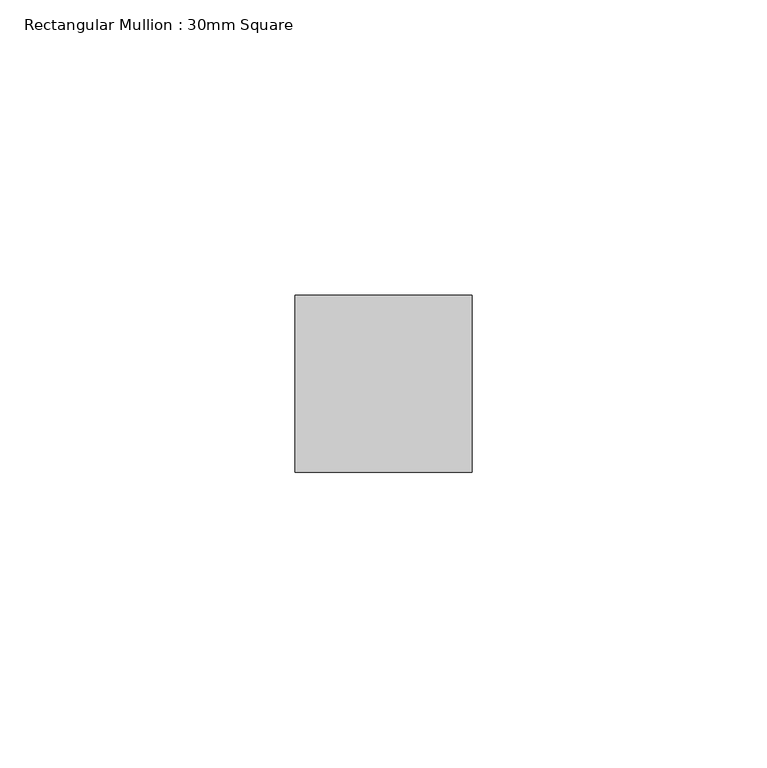
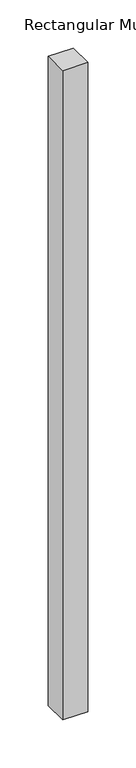
"""IFC4 building model written with IfcOpenShell, lengths in millimetres: member geometry, Rectangular Mullion : 30mm Square."""

from ifc_helpers import new_model, si_unit, frame, origin, place, context, project, spatial, polyline, outline, extrude, source, transform, mapped, element, save


def rectangular_mullion_30mm_square_b29643f7(model_context):
    return source(origin(), model_context, "Body", "SweptSolid", [
        extrude(outline(polyline([(15.0, 15.0), (15.0, -15.0), (-15.0, -15.0), (-15.0, 15.0), (15.0, 15.0)])), frame((0.0, 0.0, -823.5748774), z_axis=(0.0, 0.0, 1.0), x_axis=(1.0, 0.0, 0.0)), (0.0, 0.0, 1.0), 823.5748774),
    ])


if __name__ == "__main__":
    model = new_model("IFC4")
    model_context = context("Model", 3, world=origin())
    ifc_project = project(units=[si_unit("LENGTHUNIT", "METRE", prefix="MILLI")], contexts=[model_context])
    site = spatial("IfcSite", under=ifc_project)
    building = spatial("IfcBuilding", under=site)
    placement = place(None, origin())
    rectangular_mullion_30mm_square_shape = rectangular_mullion_30mm_square_b29643f7(model_context)
    element("IfcMember", 1, ObjectType="Rectangular Mullion : 30mm Square", at=placement, inside=building, context=model_context, shape_type="MappedRepresentation", body=[
        mapped(rectangular_mullion_30mm_square_shape, transform((0.0, 0.0, 0.0), x_axis=(1.0, 0.0, 0.0), y_axis=(0.0, 1.0, 0.0), z_axis=(0.0, 0.0, 1.0))),
    ])
    save(model, "model.ifc")

# Revit data of these elements
# Type "Rectangular Mullion : 30mm Square"
#   built-in parameter 1007304 = 0.0984252 (stored number, unit not read)
#   built-in parameter 1007301 = 0.0492126 (stored number, unit not read)
#   built-in parameter 1007300 = 0.0492126 (stored number, unit not read)
# Element 1 (IfcMember, "Rectangular Mullion : 30mm Square")
#   Materials on its faces: "Aluminum"
# Materials
#   "Aluminum": class "Metal", colour RGB 244 244 244, transparency 0, Description = "Aluminum 6061", Cost = 0
